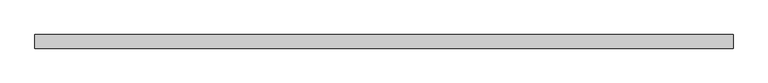
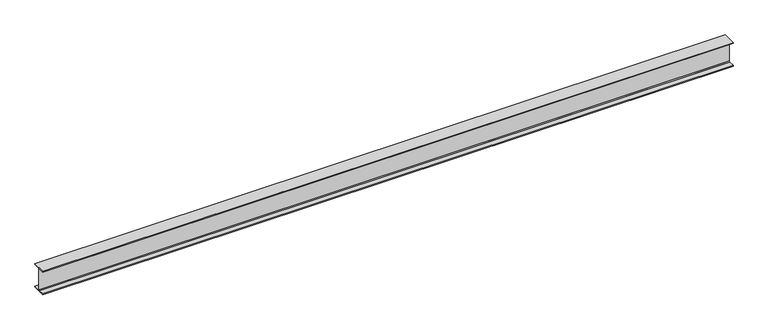
"""IFC4 building model written with IfcOpenShell, lengths in millimetres: beam geometry, Old_Steel Beam_H-KSD3502 : H_SB_ASB_H-800×300x14x26."""

from ifc_helpers import new_model, si_unit, point, frame, frame_2d, origin, place, context, project, spatial, polyline, circle_curve, trimmed, segment, composite_curve, outline, extrude, source, transform, mapped, element, save


def beam_c1ccdf6e(model_context):
    return source(origin(), model_context, "Body", "SweptSolid", [
        extrude(outline(composite_curve([segment(polyline([(82.5, -141.5), (82.5, -151.7), (-82.5, -151.7), (-82.5, -141.5), (-11.9, -141.5)]), True, "CONTINUOUS"), segment(trimmed(circle_curve(frame_2d((-11.9, -132.6)), 8.9), [point((-11.9, -141.5))], [point((-3.0, -132.6))], True, "CARTESIAN"), True, "CONTINUOUS"), segment(polyline([(-3.0, -132.6), (-3.0, 132.6)]), True, "CONTINUOUS"), segment(trimmed(circle_curve(frame_2d((-11.9, 132.6)), 8.9), [point((-3.0, 132.6))], [point((-11.9, 141.5))], True, "CARTESIAN"), True, "CONTINUOUS"), segment(polyline([(-11.9, 141.5), (-82.5, 141.5), (-82.5, 151.7), (82.5, 151.7), (82.5, 141.5), (11.9, 141.5)]), True, "CONTINUOUS"), segment(trimmed(circle_curve(frame_2d((11.9, 132.6)), 8.9), [point((11.9, 141.5))], [point((3.0, 132.6))], True, "CARTESIAN"), True, "CONTINUOUS"), segment(polyline([(3.0, 132.6), (3.0, -132.6)]), True, "CONTINUOUS"), segment(trimmed(circle_curve(frame_2d((11.9, -132.6)), 8.9), [point((3.0, -132.6))], [point((11.9, -141.5))], True, "CARTESIAN"), True, "CONTINUOUS"), segment(polyline([(11.9, -141.5), (82.5, -141.5)]), True, "CONTINUOUS")], self_intersect=False)), frame((-4157.9983828, 0.0, 0.0), z_axis=(1.0, 0.0, 0.0), x_axis=(0.0, 1.0, 0.0)), (0.0, 0.0, 1.0), 8443.8590445),
    ])


if __name__ == "__main__":
    model = new_model("IFC4")
    model_context = context("Model", 3, world=origin())
    ifc_project = project(units=[si_unit("LENGTHUNIT", "METRE", prefix="MILLI")], contexts=[model_context])
    site = spatial("IfcSite", under=ifc_project)
    building = spatial("IfcBuilding", under=site)
    placement = place(None, origin())
    beam_shape = beam_c1ccdf6e(model_context)
    element("IfcBeam", 1, ObjectType="Old_Steel Beam_H-KSD3502 : H_SB_ASB_H-800×300x14x26", at=placement, inside=building, context=model_context, shape_type="MappedRepresentation", body=[
        mapped(beam_shape, transform((0.0, 0.0, 0.0), x_axis=(1.0, 0.0, 0.0), y_axis=(0.0, 1.0, 0.0), z_axis=(0.0, 0.0, 1.0))),
    ])
    save(model, "model.ifc")

# Revit data of these elements
# Type "Old_Steel Beam_H-KSD3502 : H_SB_ASB_H-800×300x14x26"
#   Width = 30.0 cm
#   Web Thickness = 1.4 cm
#   Web Fillet = 2.8 cm
#   Warping Constant = 17523000.0 cm⁶
#   Torsional Moment of Inertia = 422.315 cm⁴
#   Torsional Modulus = 1.0 cm³
#   Section Area = 267.4 cm²
#   Plastic Modulus weak axis = 1220.0 cm³
#   Plastic Modulus strong axis = 8240.0 cm³
#   Perimeter = 2.72 m²/m
#   Nominal Weight = 210.00 kgf/m
#   Moment of Inertia weak axis = 11700.00 cm⁴
#   Moment of Inertia strong axis = 292000.00 cm⁴
#   Height = 80.0 cm
#   Flange Thickness = 2.6 cm
#   Elastic Modulus weak axis = 782.0 cm³
#   Elastic Modulus strong axis = 7290.0 cm³
#   Centroid Vertical = 40.0 cm
#   Centroid Horizontal = 15.0 cm
#   Length [instance default] = 1.5240 m
#   Structural Material [instance default] = Steel, 45-345
#   Assembly Code = ""
# Element 1 (IfcBeam, "Old_Steel Beam_H-KSD3502 : H_SB_ASB_H-800×300x14x26")
#   Structural Material = none
# Materials
#   "Steel, 45-345": class "Metal", colour RGB 189 187 185, transparency 0, Description = "Steel 345 MPa", Cost = 0
